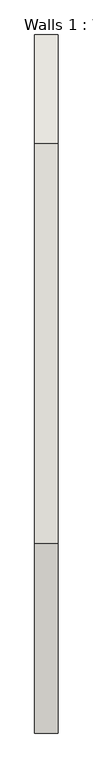
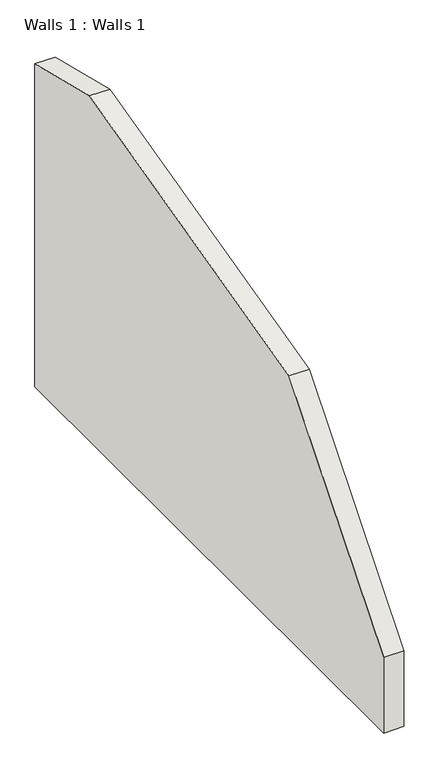
"""IFC4 building model written with IfcOpenShell, lengths in millimetres: wall geometry, Walls 1 : Walls 1."""

from ifc_helpers import new_model, si_unit, frame, origin, place, context, project, spatial, polyline, outline, extrude, source, transform, mapped, element, save


def walls_1_walls_1_2f73d3c6(model_context):
    return source(origin(), model_context, "Body", "SweptSolid", [
        extrude(outline(polyline([(7113.772024, 5648.2612183), (7913.3615366, 5448.3638401), (7913.3615366, 2559.05), (2795.1519691, 2559.05), (2795.1519691, 3237.9527527), (4186.0606359, 4916.3333713), (7113.772024, 5648.2612183)])), frame((22549.6370052, 0.0, 0.0), z_axis=(1.0, 0.0, 0.0), x_axis=(0.0, 1.0, 0.0)), (0.0, 0.0, 1.0), 171.45),
    ])


if __name__ == "__main__":
    model = new_model("IFC4")
    model_context = context("Model", 3, world=origin())
    ifc_project = project(units=[si_unit("LENGTHUNIT", "METRE", prefix="MILLI")], contexts=[model_context])
    site = spatial("IfcSite", under=ifc_project)
    building = spatial("IfcBuilding", under=site)
    placement = place(None, origin())
    walls_1_walls_1_shape = walls_1_walls_1_2f73d3c6(model_context)
    element("IfcWall", 1, ObjectType="Walls 1 : Walls 1", at=placement, inside=building, context=model_context, shape_type="MappedRepresentation", body=[
        mapped(walls_1_walls_1_shape, transform((0.0, 0.0, 0.0), x_axis=(1.0, 0.0, 0.0), y_axis=(0.0, 1.0, 0.0), z_axis=(0.0, 0.0, 1.0))),
    ])
    save(model, "model.ifc")

# Revit data of these elements
# Element 1 (IfcWall, "Walls 1 : Walls 1")
#   Materials on its faces: "Default Wall"
# Materials
#   "Default Wall": class "Miscellaneous", colour RGB 80 80 80, transparency 0
